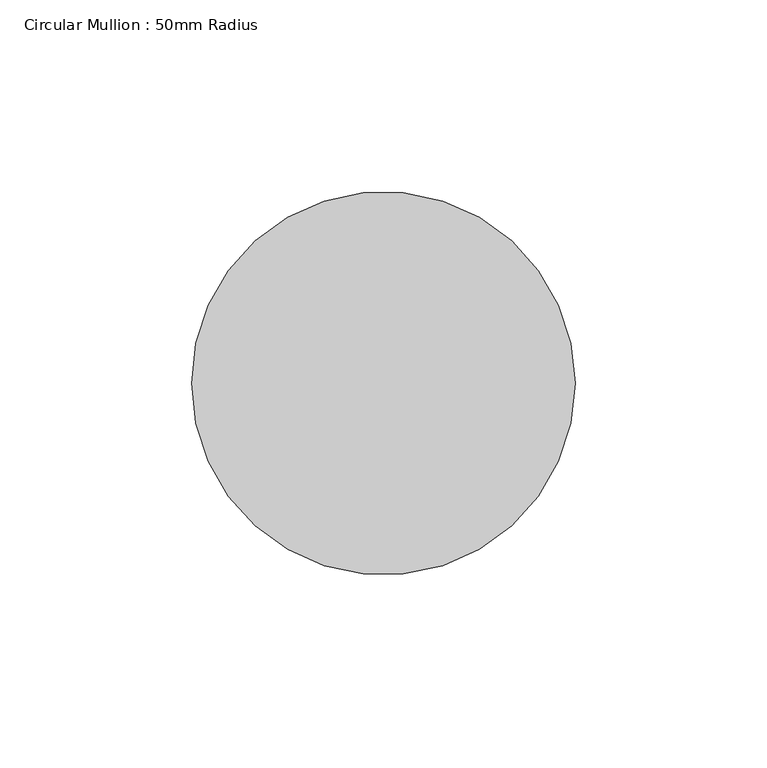
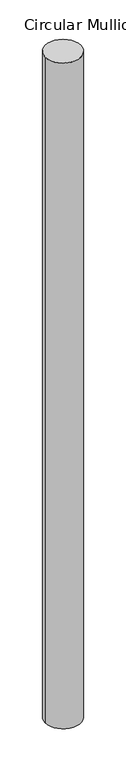
"""IFC4 building model written with IfcOpenShell, lengths in millimetres: member geometry, Circular Mullion : 50mm Radius."""

from ifc_helpers import new_model, si_unit, point, frame, origin, origin_2d, place, context, project, spatial, circle_curve, trimmed, segment, composite_curve, outline, extrude, source, transform, mapped, element, save


def circular_mullion_50mm_radius_26d8bbea(model_context):
    return source(origin(), model_context, "Body", "SweptSolid", [
        extrude(outline(composite_curve([segment(trimmed(circle_curve(origin_2d(), 50.0), [point((50.0, 0.0))], [point((-50.0, 0.0))], False, "CARTESIAN"), True, "CONTINUOUS"), segment(trimmed(circle_curve(origin_2d(), 50.0), [point((-50.0, 0.0))], [point((50.0, 0.0))], False, "CARTESIAN"), True, "CONTINUOUS")], self_intersect=False)), frame((0.0, 0.0, -1960.0553567), z_axis=(0.0, 0.0, 1.0), x_axis=(1.0, 0.0, 0.0)), (0.0, 0.0, 1.0), 1960.0553567),
    ])


if __name__ == "__main__":
    model = new_model("IFC4")
    model_context = context("Model", 3, world=origin())
    ifc_project = project(units=[si_unit("LENGTHUNIT", "METRE", prefix="MILLI")], contexts=[model_context])
    site = spatial("IfcSite", under=ifc_project)
    building = spatial("IfcBuilding", under=site)
    placement = place(None, origin())
    circular_mullion_50mm_radius_shape = circular_mullion_50mm_radius_26d8bbea(model_context)
    element("IfcMember", 1, ObjectType="Circular Mullion : 50mm Radius", at=placement, inside=building, context=model_context, shape_type="MappedRepresentation", body=[
        mapped(circular_mullion_50mm_radius_shape, transform((0.0, 0.0, 0.0), x_axis=(1.0, 0.0, 0.0), y_axis=(0.0, 1.0, 0.0), z_axis=(0.0, 0.0, 1.0))),
    ])
    save(model, "model.ifc")

# Revit data of these elements
# Type "Circular Mullion : 50mm Radius"
#   built-in parameter 1007350 = 0.164042 (stored number, unit not read)
# Element 1 (IfcMember, "Circular Mullion : 50mm Radius")
#   Materials on its faces: "Aluminium"
# Materials
#   "Aluminium": class "Metal", colour RGB 247 247 247, transparency 0, Description = "Aluminium 6061", Cost = 0
